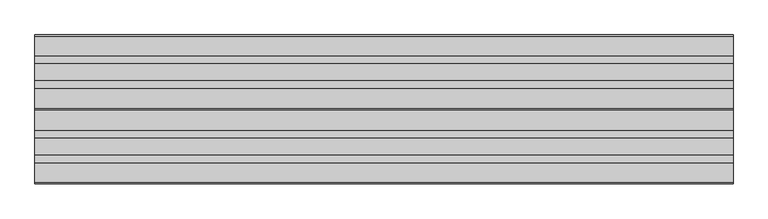
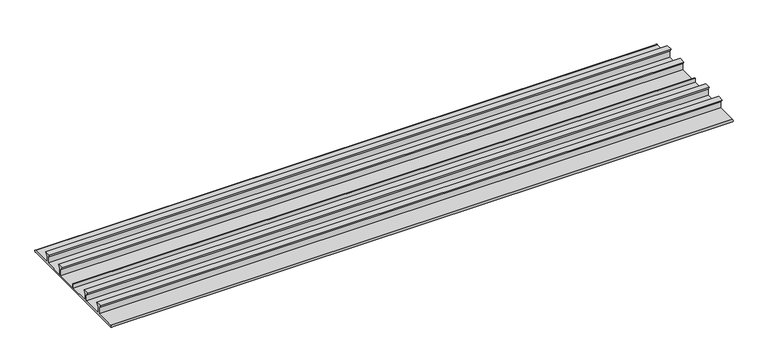
"""IFC4 building model written with IfcOpenShell, lengths in millimetres: proxy geometry, TN_ПВХ_ТПО_Гидрошпонка ТехноНИКОЛЬ : ПВХ Гидрошпонка ТехноНИКОЛЬ EC-320-4."""

from ifc_helpers import new_model, si_unit, point, frame, frame_2d, origin, place, context, project, spatial, polyline, circle_curve, trimmed, segment, composite_curve, outline, extrude, source, transform, mapped, element, save


def specialty_equipment_b3f57116(model_context):
    return source(origin(), model_context, "Body", "SweptSolid", [
        extrude(outline(composite_curve([segment(polyline([(157.5, 0.0), (-157.5, 0.0)]), True, "CONTINUOUS"), segment(trimmed(circle_curve(frame_2d((-157.5, 2.5)), 2.5), [point((-157.5, 0.0))], [point((-157.5, 5.0))], False, "CARTESIAN"), True, "CONTINUOUS"), segment(polyline([(-157.5, 5.0), (-108.7123259, 5.0), (-108.7123259, 20.0), (-114.3139862, 28.0), (-99.0193471, 28.0), (-104.6210074, 20.0), (-104.6210074, 5.0), (-55.3789926, 5.0), (-55.3789926, 20.0), (-60.9806529, 28.0), (-45.6860138, 28.0), (-51.2876741, 20.0), (-51.2876741, 5.0), (-1.032716, 5.0), (-1.032716, 15.0), (1.032716, 15.0), (1.032716, 5.0), (51.2876741, 5.0), (51.2876741, 20.0), (45.6860138, 28.0), (60.9806529, 28.0), (55.3789926, 20.0), (55.3789926, 5.0), (104.6210074, 5.0), (104.6210074, 20.0), (99.0193471, 28.0), (114.3139862, 28.0), (108.7123259, 20.0), (108.7123259, 5.0), (157.5, 5.0)]), True, "CONTINUOUS"), segment(trimmed(circle_curve(frame_2d((157.5, 2.5)), 2.5), [point((157.5, 5.0))], [point((157.5, 0.0))], False, "CARTESIAN"), True, "CONTINUOUS")], self_intersect=False)), frame((0.0, 0.0, 0.0), z_axis=(1.0, 0.0, 0.0), x_axis=(0.0, 1.0, 0.0)), (0.0, 0.0, 1.0), 1500.0),
    ])


if __name__ == "__main__":
    model = new_model("IFC4")
    model_context = context("Model", 3, world=origin())
    ifc_project = project(units=[si_unit("LENGTHUNIT", "METRE", prefix="MILLI")], contexts=[model_context])
    site = spatial("IfcSite", under=ifc_project)
    building = spatial("IfcBuilding", under=site)
    placement = place(None, origin())
    specialty_equipment_shape = specialty_equipment_b3f57116(model_context)
    element("IfcBuildingElementProxy", 1, Name="TN_ПВХ_ТПО_Гидрошпонка ТехноНИКОЛЬ : ПВХ Гидрошпонка ТехноНИКОЛЬ EC-320-4", ObjectType="TN_ПВХ_ТПО_Гидрошпонка ТехноНИКОЛЬ : ПВХ Гидрошпонка ТехноНИКОЛЬ EC-320-4", at=placement, inside=building, context=model_context, shape_type="MappedRepresentation", body=[
        mapped(specialty_equipment_shape, transform((0.0, 0.0, 0.0), x_axis=(1.0, 0.0, 0.0), y_axis=(0.0, 1.0, 0.0), z_axis=(0.0, 0.0, 1.0))),
    ])
    save(model, "model.ifc")

# Revit data of these elements
# Type "TN_ПВХ_ТПО_Гидрошпонка ТехноНИКОЛЬ : ПВХ Гидрошпонка ТехноНИКОЛЬ EC-320-4"
#   Description = "Наружная гидрошпонка применяется для герметизации рабочих швов бетонирования и для разбивки на секции (карты) гидроизоляционных систем на основе ПВХ мембран LOGICBASE V-SL"
#   Type Comments = "п.м."
#   Manufacturer = "ТехноНИКОЛЬ"
#   URL = "https://shop.tn.ru/pvh-gidroshponka-ec-320-4-15-m-rul"
#   ADSK_Примечание = ""
#   ADSK_Обозначение [instance default] = "ТехноНИКОЛЬ"
#   ADSK_Наименование = "ПВХ Гидрошпонка ТехноНИКОЛЬ EC-320-4"
#   ADSK_Масса_Текст = ""
#   ADSK_Марка = ""
#   ADSK_Код изделия = "499184"
#   ADSK_Завод-изготовитель [instance default] = "ТехноНИКОЛЬ"
#   ADSK_Единица измерения [instance default] = "п.м."
#   ADSK_Группирование = "Гидрошпонки"
#   ADSK_URL страницы изделия = "https://shop.tn.ru/pvh-gidroshponka-ec-320-4-15-m-rul"
#   ADSK_URL документации изделия = "https://nav.tn.ru/upload/iblock/67f/Katalog-i-rekomendatsii-po-primeneniyu_Gidroshponki-TEKHNONIKOL.PDF"
#   built-in parameter 1001306 [instance default] = 3.28084 (stored number, unit not read)
#   ADSK_Размер_Длина [instance default] = 1000 mm
#   ADSK_Количество [instance default] = 1
#   ПВХ_ТПО Гидрошпонка ТехноНИКОЛЬ EC-320-4 = yes
#   ПВХ Гидрошпонка ТехноНИКОЛЬ IM-260/50 = no
#   ПВХ Гидрошпонка ТехноНИКОЛЬ IM-240/20 = no
#   ПВХ Гидрошпонка ТехноНИКОЛЬ IC-240-6 = no
#   ПВХ Гидрошпонка ТехноНИКОЛЬ IC-125-2SP = no
#   ПВХ Гидрошпонка ТехноНИКОЛЬ EM-260/50 = no
#   ПВХ Гидрошпонка ТехноНИКОЛЬ EM-260/20 = no
#   ПВХ Гидрошпонка ТехноНИКОЛЬ EC-320-4 = no
#   ПВХ Гидрошпонка ТехноНИКОЛЬ EC-220-3 = no
#   ПВХ_ТПО Гидрошпонка ТехноНИКОЛЬ EC-220-3 = no
#   ПВХ Гидрошпонка ТехноНИКОЛЬ IC-240-2 = no
#   Материал = TN_ПВХ_Черный
#   Default Elevation = 0
# Element 1 (IfcBuildingElementProxy, "TN_ПВХ_ТПО_Гидрошпонка ТехноНИКОЛЬ : ПВХ Гидрошпонка ТехноНИКОЛЬ EC-320-4")
#   built-in parameter 1001306 = 4.92126 (stored number, unit not read)
#   ADSK_Размер_Длина = 1500 mm
#   ADSK_Количество = 1.5
#   Materials on its faces: "TN_ПВХ_Черный"
# Materials
#   "TN_ПВХ_Черный": class "Типовые", colour RGB 48 48 48, transparency 0, Cost = 0
